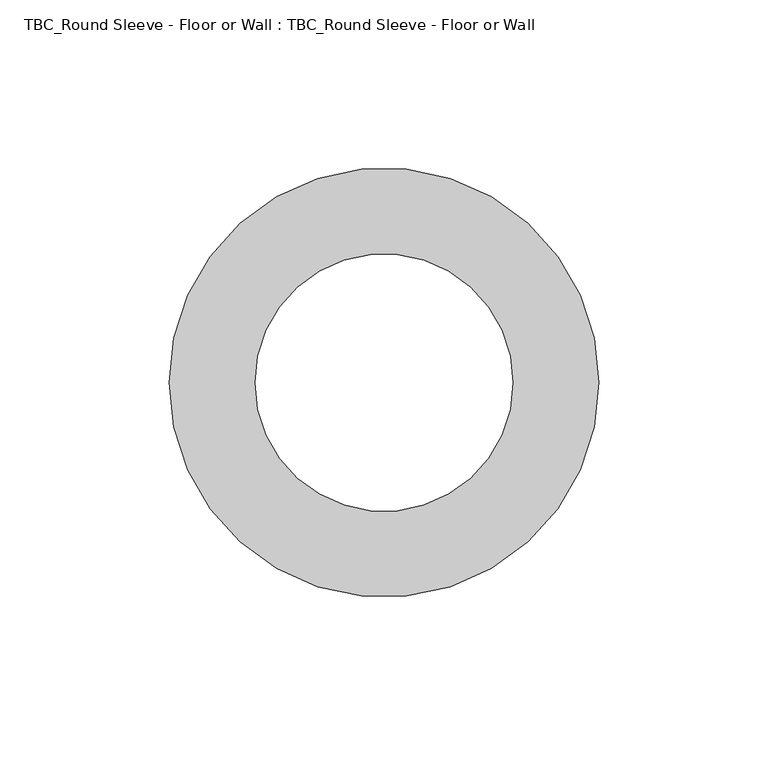
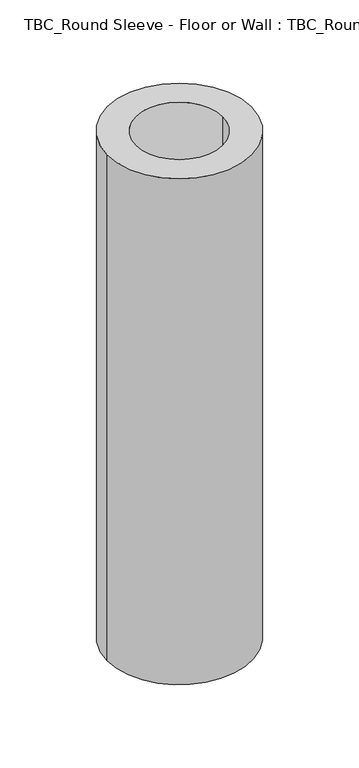
"""IFC4 building model written with IfcOpenShell, lengths in millimetres: proxy geometry, TBC_Round Sleeve - Floor or Wall : TBC_Round Sleeve - Floor or Wall."""

from ifc_helpers import new_model, si_unit, point, frame, origin, origin_2d, place, context, project, spatial, circle_curve, trimmed, segment, composite_curve, outline, extrude, source, transform, mapped, element, save


def tbc_round_sleeve_floor_or_wall_tbc_round_sleeve_floor_or_647fdbdc(model_context):
    return source(origin(), model_context, "Body", "SweptSolid", [
        extrude(outline(composite_curve([segment(trimmed(circle_curve(origin_2d(), 63.5), [point((-63.5, 0.0))], [point((63.5, 0.0))], False, "CARTESIAN"), True, "CONTINUOUS"), segment(trimmed(circle_curve(origin_2d(), 63.5), [point((63.5, 0.0))], [point((-63.5, 0.0))], False, "CARTESIAN"), True, "CONTINUOUS")], self_intersect=False), holes=[composite_curve([segment(trimmed(circle_curve(origin_2d(), 38.1), [point((-38.1, 0.0))], [point((38.1, 0.0))], True, "CARTESIAN"), True, "CONTINUOUS"), segment(trimmed(circle_curve(origin_2d(), 38.1), [point((38.1, 0.0))], [point((-38.1, 0.0))], True, "CARTESIAN"), True, "CONTINUOUS")], self_intersect=False)]), frame((0.0, 0.0, -469.9), z_axis=(0.0, 0.0, 1.0), x_axis=(1.0, 0.0, 0.0)), (0.0, 0.0, 1.0), 469.9),
    ])


if __name__ == "__main__":
    model = new_model("IFC4")
    model_context = context("Model", 3, world=origin())
    ifc_project = project(units=[si_unit("LENGTHUNIT", "METRE", prefix="MILLI")], contexts=[model_context])
    site = spatial("IfcSite", under=ifc_project)
    building = spatial("IfcBuilding", under=site)
    placement = place(None, origin())
    tbc_round_sleeve_floor_or_wall_tbc_round_sleeve_floor_or_shape = tbc_round_sleeve_floor_or_wall_tbc_round_sleeve_floor_or_647fdbdc(model_context)
    element("IfcBuildingElementProxy", 1, Name="TBC_Round Sleeve - Floor or Wall : TBC_Round Sleeve - Floor or Wall", ObjectType="TBC_Round Sleeve - Floor or Wall : TBC_Round Sleeve - Floor or Wall", at=placement, inside=building, context=model_context, shape_type="MappedRepresentation", body=[
        mapped(tbc_round_sleeve_floor_or_wall_tbc_round_sleeve_floor_or_shape, transform((0.0, 0.0, 0.0), x_axis=(1.0, 0.0, 0.0), y_axis=(0.0, 1.0, 0.0), z_axis=(0.0, 0.0, 1.0))),
    ])
    save(model, "model.ifc")

# Revit data of these elements
# Type "TBC_Round Sleeve - Floor or Wall : TBC_Round Sleeve - Floor or Wall"
#   Tag Dimension [instance default] = ""
#   MEP Type [instance default] = ""
#   MEP Element [instance default] = ""
#   MEP Category [instance default] = ""
#   Host Element Type [instance default] = ""
#   Host Element Id [instance default] = ""
#   Host Element Category [instance default] = ""
#   Control Line Y [instance default] = ""
#   Control Line X [instance default] = ""
#   Sleeve Radius [instance default] = 1' - 0"
#   Sleeve Edge [instance default] = 1' - 2"
#   Sleeve Depth [instance default] = 3' - 0"
#   Distance Y [instance default] = 0' - 0"
#   Distance X [instance default] = 0' - 0"
#   Default Elevation = 0
# Element 1 (IfcBuildingElementProxy, "TBC_Round Sleeve - Floor or Wall : TBC_Round Sleeve - Floor or Wall")
#   Sleeve Radius = 0' - 3"
#   Sleeve Edge = 0' - 5"
#   Sleeve Depth = 1' - 6 1/2"
